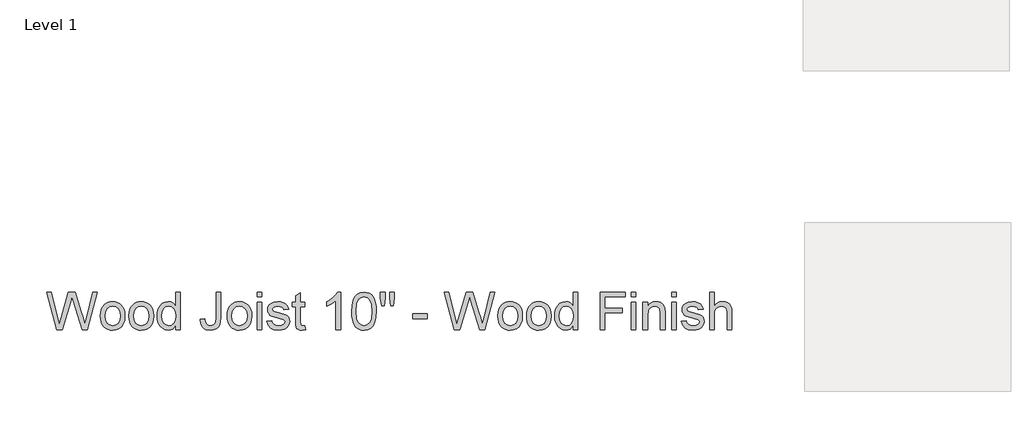
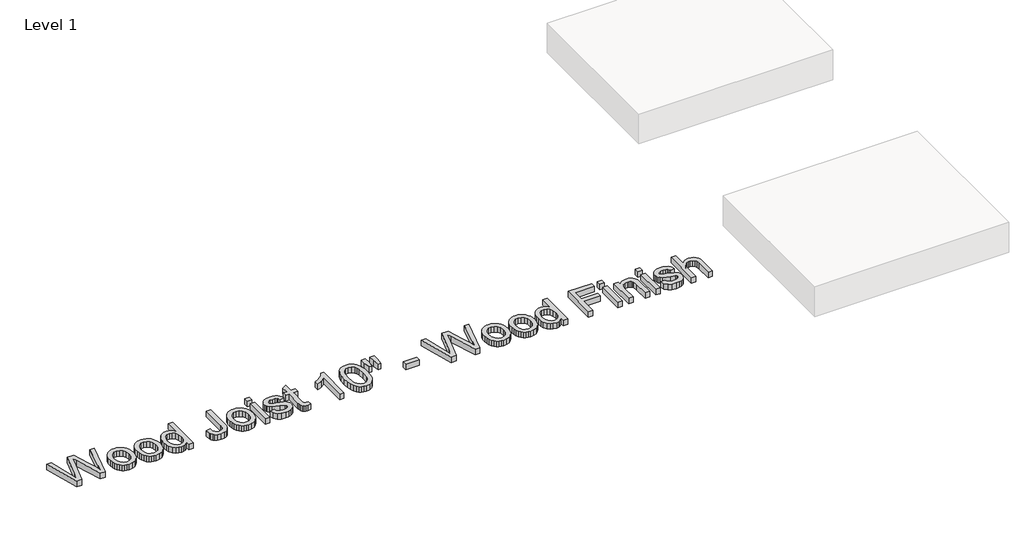
# One storey, part 14 of 42: 1 proxy.
"""IFC4 building model written with IfcOpenShell, lengths in millimetres."""

from ifc_helpers import new_model, si_unit, origin, origin_with_axes, place, context, project, spatial, polyline, outline, extrude, element, save

model = new_model("IFC4")

# Units and contexts
model_context = context("Model", 3, world=origin())
ifc_project = project(units=[si_unit("LENGTHUNIT", "METRE", prefix="MILLI")], contexts=[model_context])

# Site, building, storey
site = spatial("IfcSite", under=ifc_project)
building = spatial("IfcBuilding", under=site)
storey = spatial("IfcBuildingStorey", under=building, Name="Level 1", Elevation=0.0)

# Proxy
placement = place(None, origin())
element("IfcBuildingElementProxy", 1, Name="8\" Arial", ObjectType="8\" Arial", at=placement, inside=storey, context=model_context, shape_type="SweptSolid", body=[
    extrude(outline(polyline([(28464.8249625, -14007.0203765), (28381.7679694, -13702.4532824), (28421.0285713, -13702.4532824), (28469.2120374, -13902.6228667), (28484.0834775, -13964.4137005), (28499.9959185, -13909.7611579), (28560.3739654, -13702.4532824), (28616.9597952, -13702.4532824), (28660.8305436, -13852.729185), (28679.6243261, -13908.4970855), (28693.4733547, -13964.4137005), (28707.8986516, -13904.4074395), (28756.5282609, -13702.4532824), (28795.7888629, -13702.4532824), (28712.6575125, -14007.0203765), (28671.9841237, -14007.0203765), (28598.9653526, -13772.0516223), (28588.7784161, -13739.2600967), (28577.3274072, -13778.7437703), (28510.7777126, -14007.0203765), (28464.8249625, -14007.0203765)])), origin_with_axes(), (0.0, 0.0, 1.0), 50.8),
    extrude(outline(polyline([(28819.5831671, -13895.1871466), (28821.6419321, -13866.2203696), (28827.8182271, -13841.2595868), (28838.112052, -13820.3047982), (28852.523407, -13803.3560037), (28867.0323558, -13792.5230891), (28883.0470379, -13784.7852929), (28900.5674533, -13780.1426152), (28919.593602, -13778.5950559), (28940.5971876, -13780.4795462), (28959.5884814, -13786.1330171), (28976.5674834, -13795.5554687), (28991.5341937, -13808.7469008), (29003.7496876, -13825.2611703), (29012.4750404, -13844.6521341), (29017.710252, -13866.919792), (29019.4553226, -13892.0641442), (29016.3694987, -13930.5254062), (29007.1120273, -13959.803554), (28991.952453, -13981.7296336), (28971.1603207, -13998.134691), (28946.4644354, -14008.3681007), (28919.593602, -14011.7792373), (28898.283293, -14009.901718), (28879.1154009, -14004.26916), (28862.0899256, -13994.8815634), (28847.2068671, -13981.7389282), (28835.1214984, -13965.064326), (28826.4890921, -13945.0808283), (28821.3096483, -13921.7884352), (28819.5831671, -13895.1871466)]), holes=[polyline([(28857.6540538, -13895.1127894), (28862.059718, -13929.5680573), (28875.2767104, -13954.1152282), (28895.1672616, -13968.81007), (28919.593602, -13973.7083505), (28943.9084067, -13968.782186), (28963.7617792, -13954.0036924), (28976.9787717, -13929.1312087), (28981.3844358, -13893.9230742), (28976.9508877, -13860.4716285), (28963.6502434, -13836.2590651), (28943.7689869, -13821.5642233), (28919.593602, -13816.6659427), (28895.1672616, -13821.545634), (28875.2767104, -13836.1847079), (28862.059718, -13860.6761108), (28857.6540538, -13895.1127894)])]), origin_with_axes(), (0.0, 0.0, 1.0), 50.8),
    extrude(outline(polyline([(29052.7673485, -13895.1871466), (29054.8261135, -13866.2203696), (29061.0024085, -13841.2595868), (29071.2962334, -13820.3047982), (29085.7075884, -13803.3560037), (29100.2165372, -13792.5230891), (29116.2312193, -13784.7852929), (29133.7516347, -13780.1426152), (29152.7777834, -13778.5950559), (29173.781369, -13780.4795462), (29192.7726628, -13786.1330171), (29209.7516648, -13795.5554687), (29224.7183751, -13808.7469008), (29236.933869, -13825.2611703), (29245.6592218, -13844.6521341), (29250.8944334, -13866.919792), (29252.639504, -13892.0641442), (29249.5536801, -13930.5254062), (29240.2962087, -13959.803554), (29225.1366344, -13981.7296336), (29204.3445021, -13998.134691), (29179.6486168, -14008.3681007), (29152.7777834, -14011.7792373), (29131.4674744, -14009.901718), (29112.2995823, -14004.26916), (29095.274107, -13994.8815634), (29080.3910485, -13981.7389282), (29068.3056798, -13965.064326), (29059.6732735, -13945.0808283), (29054.4938297, -13921.7884352), (29052.7673485, -13895.1871466)]), holes=[polyline([(29090.8382352, -13895.1127894), (29095.2438994, -13929.5680573), (29108.4608918, -13954.1152282), (29128.351443, -13968.81007), (29152.7777834, -13973.7083505), (29177.0925881, -13968.782186), (29196.9459606, -13954.0036924), (29210.1629531, -13929.1312087), (29214.5686172, -13893.9230742), (29210.1350691, -13860.4716285), (29196.8344248, -13836.2590651), (29176.9531683, -13821.5642233), (29152.7777834, -13816.6659427), (29128.351443, -13821.545634), (29108.4608918, -13836.1847079), (29095.2438994, -13860.6761108), (29090.8382352, -13895.1127894)])]), origin_with_axes(), (0.0, 0.0, 1.0), 50.8),
    extrude(outline(polyline([(29433.4762161, -14007.0203765), (29433.4762161, -13971.1058485), (29422.0856224, -13988.9004561), (29408.2877143, -14001.6108901), (29392.0824919, -14009.2371505), (29373.4699551, -14011.7792373), (29348.8577217, -14008.0985559), (29326.3274899, -13997.0565116), (29307.2548679, -13979.4245604), (29293.0154639, -13955.9741582), (29284.1483678, -13927.6533594), (29281.192669, -13895.4102182), (29283.9160015, -13863.566747), (29292.0859989, -13834.8090996), (29305.6933667, -13810.7731345), (29324.72881, -13793.09471), (29347.7516583, -13782.2199694), (29373.3212407, -13778.5950559), (29391.9477195, -13781.1882633), (29408.4178394, -13788.9678854), (29422.3784039, -13800.8929215), (29433.4762161, -13815.9223707), (29433.4762161, -13702.4532824), (29471.5471028, -13702.4532824), (29471.5471028, -14007.0203765), (29433.4762161, -14007.0203765)]), holes=[polyline([(29319.2635558, -13895.2615038), (29323.5576841, -13929.6981824), (29336.4400692, -13954.1895854), (29355.1594944, -13968.8286593), (29376.9647435, -13973.7083505), (29398.760698, -13969.0517309), (29417.0060961, -13955.0818718), (29429.3586861, -13931.5385231), (29433.4762161, -13898.1614346), (29429.2843289, -13861.6706384), (29416.7086673, -13836.3706009), (29397.9985367, -13821.5921072), (29375.4032423, -13816.6659427), (29353.3749216, -13821.3969196), (29335.3247111, -13835.5898502), (29323.2788446, -13859.9697174), (29319.2635558, -13895.2615038)])]), origin_with_axes(), (0.0, 0.0, 1.0), 50.8),
    extrude(outline(polyline([(29633.3483716, -13921.5095957), (29671.4192583, -13916.6020204), (29675.3787792, -13944.2814884), (29684.4317684, -13961.5881268), (29698.2622078, -13970.6782946), (29716.5540791, -13973.7083505), (29730.6168847, -13971.9888403), (29742.616278, -13966.8303095), (29751.8737495, -13958.7067853), (29757.7107897, -13948.0922949), (29761.8376144, -13910.3560156), (29761.8376144, -13702.4532824), (29799.9085011, -13702.4532824), (29799.9085011, -13909.6868007), (29797.6127225, -13943.5843896), (29790.7253868, -13968.8379539), (29778.846824, -13987.2878343), (29761.5773642, -14000.7743716), (29739.8929455, -14009.0280209), (29714.7695063, -14011.7792373), (29679.5799611, -14006.1002061), (29665.4846242, -13999.0014171), (29653.7222445, -13989.0631125), (29644.5019517, -13976.3224709), (29638.0328752, -13960.8166709), (29633.3483716, -13921.5095957)])), origin_with_axes(), (0.0, 0.0, 1.0), 50.8),
    extrude(outline(polyline([(29852.2559704, -13895.1871466), (29854.3147354, -13866.2203696), (29860.4910304, -13841.2595868), (29870.7848554, -13820.3047982), (29885.1962103, -13803.3560037), (29899.7051591, -13792.5230891), (29915.7198412, -13784.7852929), (29933.2402566, -13780.1426152), (29952.2664054, -13778.5950559), (29973.2699909, -13780.4795462), (29992.2612847, -13786.1330171), (30009.2402867, -13795.5554687), (30024.206997, -13808.7469008), (30036.4224909, -13825.2611703), (30045.1478437, -13844.6521341), (30050.3830553, -13866.919792), (30052.1281259, -13892.0641442), (30049.0423021, -13930.5254062), (30039.7848306, -13959.803554), (30024.6252563, -13981.7296336), (30003.833124, -13998.134691), (29979.1372388, -14008.3681007), (29952.2664054, -14011.7792373), (29930.9560964, -14009.901718), (29911.7882042, -14004.26916), (29894.7627289, -13994.8815634), (29879.8796705, -13981.7389282), (29867.7943017, -13965.064326), (29859.1618954, -13945.0808283), (29853.9824517, -13921.7884352), (29852.2559704, -13895.1871466)]), holes=[polyline([(29890.3268572, -13895.1127894), (29894.7325213, -13929.5680573), (29907.9495137, -13954.1152282), (29927.8400649, -13968.81007), (29952.2664054, -13973.7083505), (29976.58121, -13968.782186), (29996.4345826, -13954.0036924), (30009.651575, -13929.1312087), (30014.0572391, -13893.9230742), (30009.623691, -13860.4716285), (29996.3230468, -13836.2590651), (29976.4417902, -13821.5642233), (29952.2664054, -13816.6659427), (29927.8400649, -13821.545634), (29907.9495137, -13836.1847079), (29894.7325213, -13860.6761108), (29890.3268572, -13895.1127894)])]), origin_with_axes(), (0.0, 0.0, 1.0), 50.8),
    extrude(outline(polyline([(30094.9578735, -14007.0203765), (30094.9578735, -13783.3539168), (30133.0287603, -13783.3539168), (30133.0287603, -14007.0203765), (30094.9578735, -14007.0203765)])), origin_with_axes(), (0.0, 0.0, 1.0), 50.8),
    extrude(outline(polyline([(30094.9578735, -13740.5241692), (30094.9578735, -13702.4532824), (30133.0287603, -13702.4532824), (30133.0287603, -13740.5241692), (30094.9578735, -13740.5241692)])), origin_with_axes(), (0.0, 0.0, 1.0), 50.8),
    extrude(outline(polyline([(30175.8585079, -13940.3963246), (30213.9293946, -13935.6374638), (30219.9337386, -13951.9216907), (30231.5520512, -13963.8932001), (30248.8586896, -13971.2545629), (30271.9280112, -13973.7083505), (30294.7184932, -13971.4590452), (30310.7424699, -13964.7111293), (30320.223013, -13954.9331574), (30323.3831941, -13943.5936843), (30320.2044237, -13933.8900696), (30310.6681127, -13926.4915281), (30271.481868, -13915.6353768), (30214.1524662, -13897.008898), (30199.6435174, -13887.6491854), (30189.1312682, -13875.2594168), (30182.7458436, -13860.6296376), (30180.6173687, -13844.5498929), (30182.3275843, -13829.7992832), (30187.4582312, -13816.1826209), (30195.5445767, -13804.2389955), (30206.1218885, -13794.5074969), (30230.3251574, -13783.242381), (30263.0795043, -13778.5950559), (30287.8590414, -13780.4632806), (30309.4040403, -13786.0679546), (30326.7292681, -13794.8606936), (30338.8494918, -13806.2931132), (30346.8800695, -13821.2110266), (30351.9363591, -13840.4602469), (30313.8654724, -13845.2191077), (30309.0601383, -13833.2383038), (30299.5517112, -13824.2131985), (30285.2472447, -13818.5527566), (30266.0537923, -13816.6659427), (30244.1927753, -13818.4691048), (30229.618764, -13823.8785911), (30221.4208826, -13831.6860972), (30218.6882555, -13840.6833185), (30223.2240447, -13851.7625414), (30237.42627, -13860.1649051), (30270.2177956, -13868.26984), (30326.0972319, -13886.1899253), (30340.8571362, -13894.7595927), (30352.0478949, -13906.4894411), (30359.1025343, -13921.4166492), (30361.4540808, -13939.5783954), (30358.6935697, -13958.3535886), (30350.4120365, -13976.0134238), (30336.9254992, -13991.1729981), (30318.549976, -14002.4474086), (30296.3543516, -14009.4462801), (30271.4075108, -14011.7792373), (30233.0206059, -14007.2806267), (30205.0065305, -13993.7847947), (30186.3056946, -13971.4404559), (30175.8585079, -13940.3963246)])), origin_with_axes(), (0.0, 0.0, 1.0), 50.8),
    extrude(outline(polyline([(30485.1844628, -13975.2698518), (30489.9433236, -14008.1357345), (30461.4645158, -14011.7792373), (30443.1912337, -14010.1991468), (30429.5652767, -14005.4588752), (30419.9360192, -13998.1532803), (30413.6528357, -13988.8772195), (30410.1952259, -13972.9461892), (30409.0426893, -13945.6756859), (30409.0426893, -13821.4248035), (30380.4895242, -13821.4248035), (30380.4895242, -13783.3539168), (30409.0426893, -13783.3539168), (30409.0426893, -13728.998803), (30447.113576, -13706.6172856), (30447.113576, -13783.3539168), (30485.1844628, -13783.3539168), (30485.1844628, -13821.4248035), (30447.113576, -13821.4248035), (30447.113576, -13944.5603279), (30449.1212204, -13964.1906289), (30455.6274755, -13971.1430271), (30468.602807, -13973.7083505), (30485.1844628, -13975.2698518)])), origin_with_axes(), (0.0, 0.0, 1.0), 50.8),
    extrude(outline(polyline([(30775.4749743, -14007.0203765), (30737.4040875, -14007.0203765), (30737.4040875, -13769.6721918), (30701.3408452, -13795.3626047), (30661.262314, -13814.5839411), (30661.262314, -13778.5950559), (30691.1632034, -13762.3294183), (30717.0673932, -13742.9779568), (30737.4877394, -13722.3996015), (30750.9370981, -13702.4532824), (30775.4749743, -13702.4532824), (30775.4749743, -14007.0203765)])), origin_with_axes(), (0.0, 0.0, 1.0), 50.8),
    extrude(outline(polyline([(30865.8933304, -13857.1906171), (30868.69102, -13808.4401773), (30877.0840891, -13769.560656), (30890.9888856, -13739.9571955), (30910.3217578, -13719.0349382), (30935.2221254, -13706.5986963), (30965.8294081, -13702.4532824), (30989.2891049, -13704.90707), (31010.2950141, -13712.2684329), (31027.8619028, -13724.2492369), (31041.004538, -13740.5613478), (31050.9312243, -13761.0653458), (31058.8502662, -13785.6218114), (31064.0366809, -13816.8053624), (31065.7654858, -13857.1906171), (31062.9956801, -13905.6622173), (31054.6862629, -13944.4487921), (31040.8651183, -13974.0801366), (31021.56013, -13995.0860458), (30996.6039945, -14007.6059394), (30965.8294081, -14011.7792373), (30944.8606775, -14009.9667805), (30926.2713773, -14004.5294102), (30910.0615076, -13995.4671264), (30896.2310682, -13982.779929), (30882.9583079, -13959.8453799), (30873.4777648, -13931.2689783), (30867.789439, -13897.050724), (30865.8933304, -13857.1906171)]), holes=[polyline([(30903.9642171, -13857.1162599), (30908.4256492, -13917.0016904), (30914.0024392, -13937.4847755), (30921.8099453, -13951.6614405), (30941.7376751, -13968.196623), (30965.8294081, -13973.7083505), (30989.9211411, -13968.1780337), (31009.8488709, -13951.5870833), (31017.656377, -13937.3871817), (31023.233167, -13916.9087439), (31027.6945991, -13857.1162599), (31023.3818814, -13798.5785536), (31017.9909844, -13778.1628547), (31010.4437285, -13763.6492586), (30990.5531773, -13746.3054415), (30965.3832649, -13740.5241692), (30941.5517821, -13745.6176374), (30922.4048029, -13760.8980421), (30914.3370466, -13776.6989473), (30908.5743636, -13798.0022853), (30903.9642171, -13857.1162599)])]), origin_with_axes(), (0.0, 0.0, 1.0), 50.8),
    extrude(outline(polyline([(31108.3721618, -13811.9070818), (31099.0775118, -13753.0905361), (31099.0775118, -13702.4532824), (31137.1483985, -13702.4532824), (31137.1483985, -13753.0905361), (31128.820392, -13811.9070818), (31108.3721618, -13811.9070818)])), origin_with_axes(), (0.0, 0.0, 1.0), 50.8),
    extrude(outline(polyline([(31184.2908638, -13811.9070818), (31175.2192853, -13753.0905361), (31175.2192853, -13702.4532824), (31213.290172, -13702.4532824), (31213.290172, -13753.0905361), (31204.3673079, -13811.9070818), (31184.2908638, -13811.9070818)])), origin_with_axes(), (0.0, 0.0, 1.0), 50.8),
    extrude(outline(polyline([(31360.8148582, -13916.6020204), (31360.8148582, -13878.5311337), (31479.7863793, -13878.5311337), (31479.7863793, -13916.6020204), (31360.8148582, -13916.6020204)])), origin_with_axes(), (0.0, 0.0, 1.0), 50.8),
    extrude(outline(polyline([(31700.850337, -14007.0203765), (31617.7933438, -13702.4532824), (31657.0539458, -13702.4532824), (31705.2374119, -13902.6228667), (31720.108852, -13964.4137005), (31736.021293, -13909.7611579), (31796.3993399, -13702.4532824), (31852.9851697, -13702.4532824), (31896.8559181, -13852.729185), (31915.6497005, -13908.4970855), (31929.4987292, -13964.4137005), (31943.9240261, -13904.4074395), (31992.5536354, -13702.4532824), (32031.8142373, -13702.4532824), (31948.682887, -14007.0203765), (31908.0094982, -14007.0203765), (31834.9907271, -13772.0516223), (31824.8037906, -13739.2600967), (31813.3527817, -13778.7437703), (31746.8030871, -14007.0203765), (31700.850337, -14007.0203765)])), origin_with_axes(), (0.0, 0.0, 1.0), 50.8),
    extrude(outline(polyline([(32055.6085416, -13895.1871466), (32057.6673066, -13866.2203696), (32063.8436015, -13841.2595868), (32074.1374265, -13820.3047982), (32088.5487815, -13803.3560037), (32103.0577303, -13792.5230891), (32119.0724124, -13784.7852929), (32136.5928278, -13780.1426152), (32155.6189765, -13778.5950559), (32176.622562, -13780.4795462), (32195.6138558, -13786.1330171), (32212.5928579, -13795.5554687), (32227.5595682, -13808.7469008), (32239.7750621, -13825.2611703), (32248.5004148, -13844.6521341), (32253.7356265, -13866.919792), (32255.480697, -13892.0641442), (32252.3948732, -13930.5254062), (32243.1374017, -13959.803554), (32227.9778274, -13981.7296336), (32207.1856952, -13998.134691), (32182.4898099, -14008.3681007), (32155.6189765, -14011.7792373), (32134.3086675, -14009.901718), (32115.1407754, -14004.26916), (32098.1153001, -13994.8815634), (32083.2322416, -13981.7389282), (32071.1468728, -13965.064326), (32062.5144666, -13945.0808283), (32057.3350228, -13921.7884352), (32055.6085416, -13895.1871466)]), holes=[polyline([(32093.6794283, -13895.1127894), (32098.0850925, -13929.5680573), (32111.3020849, -13954.1152282), (32131.1926361, -13968.81007), (32155.6189765, -13973.7083505), (32179.9337811, -13968.782186), (32199.7871537, -13954.0036924), (32213.0041461, -13929.1312087), (32217.4098103, -13893.9230742), (32212.9762622, -13860.4716285), (32199.6756179, -13836.2590651), (32179.7943614, -13821.5642233), (32155.6189765, -13816.6659427), (32131.1926361, -13821.545634), (32111.3020849, -13836.1847079), (32098.0850925, -13860.6761108), (32093.6794283, -13895.1127894)])]), origin_with_axes(), (0.0, 0.0, 1.0), 50.8),
    extrude(outline(polyline([(32288.792723, -13895.1871466), (32290.851488, -13866.2203696), (32297.0277829, -13841.2595868), (32307.3216079, -13820.3047982), (32321.7329629, -13803.3560037), (32336.2419117, -13792.5230891), (32352.2565938, -13784.7852929), (32369.7770092, -13780.1426152), (32388.8031579, -13778.5950559), (32409.8067434, -13780.4795462), (32428.7980372, -13786.1330171), (32445.7770393, -13795.5554687), (32460.7437496, -13808.7469008), (32472.9592435, -13825.2611703), (32481.6845962, -13844.6521341), (32486.9198079, -13866.919792), (32488.6648784, -13892.0641442), (32485.5790546, -13930.5254062), (32476.3215831, -13959.803554), (32461.1620088, -13981.7296336), (32440.3698766, -13998.134691), (32415.6739913, -14008.3681007), (32388.8031579, -14011.7792373), (32367.4928489, -14009.901718), (32348.3249568, -14004.26916), (32331.2994815, -13994.8815634), (32316.416423, -13981.7389282), (32304.3310542, -13965.064326), (32295.698648, -13945.0808283), (32290.5192042, -13921.7884352), (32288.792723, -13895.1871466)]), holes=[polyline([(32326.8636097, -13895.1127894), (32331.2692739, -13929.5680573), (32344.4862663, -13954.1152282), (32364.3768175, -13968.81007), (32388.8031579, -13973.7083505), (32413.1179625, -13968.782186), (32432.9713351, -13954.0036924), (32446.1883275, -13929.1312087), (32450.5939917, -13893.9230742), (32446.1604436, -13860.4716285), (32432.8597993, -13836.2590651), (32412.9785428, -13821.5642233), (32388.8031579, -13816.6659427), (32364.3768175, -13821.545634), (32344.4862663, -13836.1847079), (32331.2692739, -13860.6761108), (32326.8636097, -13895.1127894)])]), origin_with_axes(), (0.0, 0.0, 1.0), 50.8),
    extrude(outline(polyline([(32669.5015905, -14007.0203765), (32669.5015905, -13971.1058485), (32658.1109969, -13988.9004561), (32644.3130888, -14001.6108901), (32628.1078664, -14009.2371505), (32609.4953296, -14011.7792373), (32584.8830961, -14008.0985559), (32562.3528643, -13997.0565116), (32543.2802424, -13979.4245604), (32529.0408384, -13955.9741582), (32520.1737422, -13927.6533594), (32517.2180435, -13895.4102182), (32519.941376, -13863.566747), (32528.1113734, -13834.8090996), (32541.7187411, -13810.7731345), (32560.7541845, -13793.09471), (32583.7770328, -13782.2199694), (32609.3466152, -13778.5950559), (32627.973094, -13781.1882633), (32644.4432139, -13788.9678854), (32658.4037783, -13800.8929215), (32669.5015905, -13815.9223707), (32669.5015905, -13702.4532824), (32707.5724773, -13702.4532824), (32707.5724773, -14007.0203765), (32669.5015905, -14007.0203765)]), holes=[polyline([(32555.2889303, -13895.2615038), (32559.5830586, -13929.6981824), (32572.4654436, -13954.1895854), (32591.1848689, -13968.8286593), (32612.990118, -13973.7083505), (32634.7860725, -13969.0517309), (32653.0314706, -13955.0818718), (32665.3840606, -13931.5385231), (32669.5015905, -13898.1614346), (32665.3097034, -13861.6706384), (32652.7340418, -13836.3706009), (32634.0239112, -13821.5921072), (32611.4286168, -13816.6659427), (32589.4002961, -13821.3969196), (32571.3500856, -13835.5898502), (32559.3042191, -13859.9697174), (32555.2889303, -13895.2615038)])]), origin_with_axes(), (0.0, 0.0, 1.0), 50.8),
    extrude(outline(polyline([(32888.4091894, -14007.0203765), (32888.4091894, -13702.4532824), (33093.0402057, -13702.4532824), (33093.0402057, -13740.5241692), (32926.4800762, -13740.5241692), (32926.4800762, -13830.9425252), (33069.2459015, -13830.9425252), (33069.2459015, -13869.013412), (32926.4800762, -13869.013412), (32926.4800762, -14007.0203765), (32888.4091894, -14007.0203765)])), origin_with_axes(), (0.0, 0.0, 1.0), 50.8),
    extrude(outline(polyline([(33140.6288142, -13740.5241692), (33140.6288142, -13702.4532824), (33178.6997009, -13702.4532824), (33178.6997009, -13740.5241692), (33140.6288142, -13740.5241692)])), origin_with_axes(), (0.0, 0.0, 1.0), 50.8),
    extrude(outline(polyline([(33140.6288142, -14007.0203765), (33140.6288142, -13783.3539168), (33178.6997009, -13783.3539168), (33178.6997009, -14007.0203765), (33140.6288142, -14007.0203765)])), origin_with_axes(), (0.0, 0.0, 1.0), 50.8),
    extrude(outline(polyline([(33235.8060311, -14007.0203765), (33235.8060311, -13783.3539168), (33273.8769178, -13783.3539168), (33273.8769178, -13814.5839411), (33287.1032049, -13798.8388038), (33302.9877619, -13787.5922772), (33321.5305888, -13780.8443612), (33342.7316857, -13778.5950559), (33361.4975842, -13780.4075127), (33378.6833922, -13785.844883), (33393.0157427, -13794.2286574), (33403.2212685, -13804.8803264), (33414.6350988, -13832.8758124), (33416.6427432, -13869.6826268), (33416.6427432, -14007.0203765), (33378.5718564, -14007.0203765), (33378.5718564, -13874.8132736), (33374.1847816, -13841.1294617), (33368.1153751, -13831.1005343), (33358.6813052, -13823.3209121), (33346.5889655, -13818.329685), (33332.5447492, -13816.6659427), (33310.2468836, -13820.402392), (33291.2393242, -13831.61174), (33283.6432714, -13840.762323), (33278.2175194, -13853.2682747), (33273.8769178, -13888.3462841), (33273.8769178, -14007.0203765), (33235.8060311, -14007.0203765)])), origin_with_axes(), (0.0, 0.0, 1.0), 50.8),
    extrude(outline(polyline([(33468.9902125, -13740.5241692), (33468.9902125, -13702.4532824), (33507.0610992, -13702.4532824), (33507.0610992, -13740.5241692), (33468.9902125, -13740.5241692)])), origin_with_axes(), (0.0, 0.0, 1.0), 50.8),
    extrude(outline(polyline([(33468.9902125, -14007.0203765), (33468.9902125, -13783.3539168), (33507.0610992, -13783.3539168), (33507.0610992, -14007.0203765), (33468.9902125, -14007.0203765)])), origin_with_axes(), (0.0, 0.0, 1.0), 50.8),
    extrude(outline(polyline([(33549.8908468, -13940.3963246), (33587.9617336, -13935.6374638), (33593.9660776, -13951.9216907), (33605.5843902, -13963.8932001), (33622.8910286, -13971.2545629), (33645.9603501, -13973.7083505), (33668.7508322, -13971.4590452), (33684.7748089, -13964.7111293), (33694.255352, -13954.9331574), (33697.415533, -13943.5936843), (33694.2367627, -13933.8900696), (33684.7004517, -13926.4915281), (33645.5142069, -13915.6353768), (33588.1848052, -13897.008898), (33573.6758564, -13887.6491854), (33563.1636072, -13875.2594168), (33556.7781826, -13860.6296376), (33554.6497077, -13844.5498929), (33556.3599233, -13829.7992832), (33561.4905701, -13816.1826209), (33569.5769157, -13804.2389955), (33580.1542275, -13794.5074969), (33604.3574963, -13783.242381), (33637.1118433, -13778.5950559), (33661.8913804, -13780.4632806), (33683.4363793, -13786.0679546), (33700.7616071, -13794.8606936), (33712.8818308, -13806.2931132), (33720.9124084, -13821.2110266), (33725.9686981, -13840.4602469), (33687.8978113, -13845.2191077), (33683.0924772, -13833.2383038), (33673.5840502, -13824.2131985), (33659.2795837, -13818.5527566), (33640.0861313, -13816.6659427), (33618.2251143, -13818.4691048), (33603.6511029, -13823.8785911), (33595.4532216, -13831.6860972), (33592.7205944, -13840.6833185), (33597.2563837, -13851.7625414), (33611.458609, -13860.1649051), (33644.2501345, -13868.26984), (33700.1295709, -13886.1899253), (33714.8894752, -13894.7595927), (33726.0802339, -13906.4894411), (33733.1348733, -13921.4166492), (33735.4864198, -13939.5783954), (33732.7259087, -13958.3535886), (33724.4443755, -13976.0134238), (33710.9578382, -13991.1729981), (33692.582315, -14002.4474086), (33670.3866906, -14009.4462801), (33645.4398497, -14011.7792373), (33607.0529449, -14007.2806267), (33579.0388695, -13993.7847947), (33560.3380335, -13971.4404559), (33549.8908468, -13940.3963246)])), origin_with_axes(), (0.0, 0.0, 1.0), 50.8),
    extrude(outline(polyline([(33778.3161674, -14007.0203765), (33778.3161674, -13702.4532824), (33816.3870541, -13702.4532824), (33816.3870541, -13814.4352266), (33830.3708552, -13798.755152), (33846.0741665, -13787.5550986), (33863.4969881, -13780.8350666), (33882.63932, -13778.5950559), (33905.6342843, -13781.0395489), (33925.3947104, -13788.3730278), (33940.9539546, -13800.0192244), (33951.3453734, -13815.4018703), (33957.201003, -13836.5379046), (33959.1528795, -13865.4442663), (33959.1528795, -14007.0203765), (33921.0819927, -14007.0203765), (33921.0819927, -13869.385198), (33918.0519368, -13845.5537151), (33908.961769, -13829.2323096), (33894.3134005, -13819.8075344), (33874.6087423, -13816.6659427), (33858.519703, -13818.7851229), (33843.4158966, -13825.1426636), (33830.9052976, -13835.1251177), (33822.5958804, -13848.1190386), (33817.9392607, -13865.3884984), (33816.3870541, -13888.1975697), (33816.3870541, -14007.0203765), (33778.3161674, -14007.0203765)])), origin_with_axes(), (0.0, 0.0, 1.0), 50.8),
])

save(model, "model.ifc")

# Revit data of these elements
# Element 1 (IfcBuildingElementProxy, "8\" Arial")
#   Phase Created = New Construction
